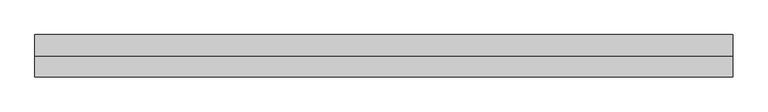
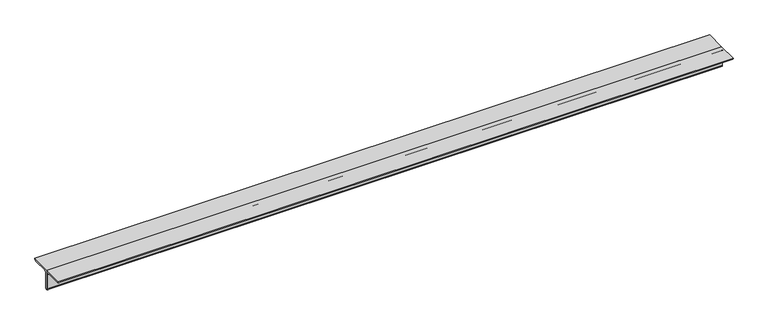
"""IFC4 building model written with IfcOpenShell, lengths in millimetres: member geometry, 0123_Steel Framing_2Ls-KSD3502 : H_SB_AR_S03_2Ls-130x130x12_HBR4."""

import ifcopenshell
import ifcopenshell.guid

model = None  # the IFC model being written
_history = None  # IfcOwnerHistory: only IFC2X3 demands one
_inside = {}  # id of a spatial element -> (the spatial element, [elements in it])
_under = {}  # id of a project, library or spatial element -> (it, [spatial elements below it])
_declared = {}  # id of a project -> (the project, [libraries it declares])
_typed = {}  # id of a type object -> (the type object, [elements of that type])
_made_of = {}  # id of a material, layer set ... -> (it, [elements and type objects made of it])


def new_model(schema):
    """Start an empty IFC model of exactly this schema.

    Asked for "IFC4X3", IfcOpenShell would pick the latest addendum, in which some entities
    have other attributes; the version numbers below select the first issue.
    IFC2X3 requires an IfcOwnerHistory on every rooted entity: one is made here for all.
    """
    global model, _history
    if schema == "IFC4X3":
        model = ifcopenshell.file(schema_version=(4, 3, 0, 0))
    else:
        model = ifcopenshell.file(schema=schema)
    _inside.clear()
    _under.clear()
    _declared.clear()
    _typed.clear()
    _made_of.clear()
    _history = None
    if model.schema == "IFC2X3":
        org = make("IfcOrganization", Name="unknown")
        user = make(
            "IfcPersonAndOrganization",
            ThePerson=make("IfcPerson", FamilyName="unknown"),
            TheOrganization=org,
        )
        app = make(
            "IfcApplication",
            ApplicationDeveloper=org,
            Version="unknown",
            ApplicationFullName="unknown",
            ApplicationIdentifier="unknown",
        )
        _history = make(
            "IfcOwnerHistory",
            OwningUser=user,
            OwningApplication=app,
            ChangeAction="ADDED",
            CreationDate=0,
        )
    return model


def make(cls, **values):
    """One entity of the class cls with the attributes given. An attribute that is None is left unset."""
    return model.create_entity(
        cls, **{name: value for name, value in values.items() if value is not None}
    )


def rooted(cls, **values):
    """An entity with a GlobalId (a new one), such as an element, a storey or a relation."""
    return make(cls, GlobalId=ifcopenshell.guid.new(), OwnerHistory=_history, **values)


def si_unit(unit_type, name, prefix=None):
    """IfcSIUnit, for example si_unit("LENGTHUNIT", "METRE", prefix="MILLI")."""
    return make("IfcSIUnit", UnitType=unit_type, Prefix=prefix, Name=name)


def assignment(units):
    """IfcUnitAssignment: the units of a project."""
    return None if units is None else make("IfcUnitAssignment", Units=units)


def point(xyz):
    """IfcCartesianPoint."""
    return None if xyz is None else make("IfcCartesianPoint", Coordinates=xyz)


def direction(xyz):
    """IfcDirection."""
    return None if xyz is None else make("IfcDirection", DirectionRatios=xyz)


def frame(location, z_axis=None, x_axis=None):
    """IfcAxis2Placement3D, a coordinate frame: its origin and axes. An axis left out is left unset."""
    return make(
        "IfcAxis2Placement3D",
        Location=point(location),
        Axis=direction(z_axis),
        RefDirection=direction(x_axis),
    )


def frame_2d(location, x_axis=None):
    """IfcAxis2Placement2D, a coordinate frame in the plane: its origin and x axis."""
    return make(
        "IfcAxis2Placement2D", Location=point(location), RefDirection=direction(x_axis)
    )


def origin():
    """The frame at (0, 0, 0) with its axes left unset."""
    return frame((0.0, 0.0, 0.0))


def place(relative_to, where):
    """IfcLocalPlacement: puts the frame where relative to a parent placement (None: the world)."""
    return make(
        "IfcLocalPlacement", PlacementRelTo=relative_to, RelativePlacement=where
    )


def context(
    kind, dimensions, precision=None, world=None, true_north=None, identifier=None
):
    """IfcGeometricRepresentationContext, for example the 3D "Model" context."""
    return make(
        "IfcGeometricRepresentationContext",
        ContextIdentifier=identifier,
        ContextType=kind,
        CoordinateSpaceDimension=dimensions,
        Precision=precision,
        WorldCoordinateSystem=world,
        TrueNorth=true_north,
    )


def project(units=None, contexts=None):
    """IfcProject with its units and contexts."""
    return rooted(
        "IfcProject",
        Name="project",
        RepresentationContexts=contexts,
        UnitsInContext=assignment(units),
    )


def spatial(cls, under=None, at=None, **own):
    """A site, building, storey or space (cls), placed at a placement, below another one or the project."""
    s = rooted(cls, ObjectPlacement=at, **own)
    if under is not None:
        _under.setdefault(under.id(), (under, []))[1].append(s)
    return s


def polyline(points):
    """IfcPolyline through the points."""
    return make("IfcPolyline", Points=[point(p) for p in points])


def circle_curve(where, radius):
    """IfcCircle in the frame where."""
    return make("IfcCircle", Position=where, Radius=radius)


def trimmed(basis, trim1, trim2, sense, master):
    """IfcTrimmedCurve: the piece of a basis curve between two trims."""
    return make(
        "IfcTrimmedCurve",
        BasisCurve=basis,
        Trim1=trim1,
        Trim2=trim2,
        SenseAgreement=sense,
        MasterRepresentation=master,
    )


def segment(curve, same_sense, transition):
    """IfcCompositeCurveSegment."""
    return make(
        "IfcCompositeCurveSegment",
        Transition=transition,
        SameSense=same_sense,
        ParentCurve=curve,
    )


def composite_curve(segments, self_intersect=None):
    """IfcCompositeCurve: segments joined end to end."""
    return make("IfcCompositeCurve", Segments=segments, SelfIntersect=self_intersect)


def outline(outer, holes=None, kind="AREA"):
    """IfcArbitraryClosedProfileDef: a profile drawn as a closed curve; with holes, ...WithVoids."""
    if holes is None:
        return make("IfcArbitraryClosedProfileDef", ProfileType=kind, OuterCurve=outer)
    return make(
        "IfcArbitraryProfileDefWithVoids",
        ProfileType=kind,
        OuterCurve=outer,
        InnerCurves=holes,
    )


def extrude(swept, where, along, depth):
    """IfcExtrudedAreaSolid: the profile swept, set in the frame where, extruded along a direction by depth."""
    return make(
        "IfcExtrudedAreaSolid",
        SweptArea=swept,
        Position=where,
        ExtrudedDirection=direction(along),
        Depth=depth,
    )


def shape(context_of_items, identifier, shape_type, items):
    """IfcShapeRepresentation: the items that make up one representation, for example the "Body"."""
    return make(
        "IfcShapeRepresentation",
        ContextOfItems=context_of_items,
        RepresentationIdentifier=identifier,
        RepresentationType=shape_type,
        Items=items,
    )


def source(mapping_origin, context_of_items, identifier, shape_type, items):
    """IfcRepresentationMap: a shape defined once, which mapped items show again and again."""
    return make(
        "IfcRepresentationMap",
        MappingOrigin=mapping_origin,
        MappedRepresentation=shape(context_of_items, identifier, shape_type, items),
    )


def transform(
    local_origin,
    x_axis=None,
    y_axis=None,
    z_axis=None,
    scale=None,
    scale2=None,
    scale3=None,
    uniform=True,
):
    """IfcCartesianTransformationOperator3D, or its non-uniform kind. x_axis, y_axis, z_axis: its Axis1, 2, 3."""
    if uniform:
        return make(
            "IfcCartesianTransformationOperator3D",
            Axis1=direction(x_axis),
            Axis2=direction(y_axis),
            LocalOrigin=point(local_origin),
            Scale=scale,
            Axis3=direction(z_axis),
        )
    return make(
        "IfcCartesianTransformationOperator3DnonUniform",
        Axis1=direction(x_axis),
        Axis2=direction(y_axis),
        LocalOrigin=point(local_origin),
        Scale=scale,
        Axis3=direction(z_axis),
        Scale2=scale2,
        Scale3=scale3,
    )


def mapped(mapping_source, mapping_target):
    """IfcMappedItem: shows the shape of a source again, moved by a transform."""
    return make(
        "IfcMappedItem", MappingSource=mapping_source, MappingTarget=mapping_target
    )


def made_of(thing, what):
    """Note that an element or type object is made of a material, layer set ...; save() writes the relation."""
    if what is not None:
        _made_of.setdefault(what.id(), (what, []))[1].append(thing)
    return thing


def element(
    cls,
    number,
    at=None,
    inside=None,
    cuts=None,
    type_object=None,
    material=None,
    context=None,
    identifier="Body",
    shape_type=None,
    held_by="IfcProductDefinitionShape",
    body=None,
    shapes=None,
    **own,
):
    """One element of the class cls, such as IfcWall. Its Tag is "e" and its number.

    at: its placement. inside: the storey or other place that contains it. cuts: it is an
    opening in that element (IfcRelVoidsElement). A single representation is given by context,
    identifier, shape_type and body (its items); several are given by shapes. held_by: the class
    of the entity that holds the representations. save() writes the other relations.
    """
    e = rooted(cls, Tag="e%d" % number, ObjectPlacement=at, **own)
    if body is not None:
        shapes = [shape(context, identifier, shape_type, body)]
    if shapes is not None:
        e.Representation = make(held_by, Representations=shapes)
    if inside is not None:
        _inside.setdefault(inside.id(), (inside, []))[1].append(e)
    if cuts is not None:
        rooted(
            "IfcRelVoidsElement", RelatingBuildingElement=cuts, RelatedOpeningElement=e
        )
    if type_object is not None:
        _typed.setdefault(type_object.id(), (type_object, []))[1].append(e)
    return made_of(e, material)


def aggregate(whole, parts):
    """IfcRelAggregates: a whole, such as a stair, and the parts it consists of."""
    return rooted("IfcRelAggregates", RelatingObject=whole, RelatedObjects=parts)


def save(model, path):
    """Write the relations noted so far, then the file.

    IfcRelAggregates (storeys below a building ...), IfcRelContainedInSpatialStructure (elements
    in a storey), IfcRelDefinesByType, IfcRelAssociatesMaterial and IfcRelDeclares: one each for
    every whole, place, type object, material and project.
    """
    for whole, parts in _under.values():
        aggregate(whole, parts)
    for where, things in _inside.values():
        rooted(
            "IfcRelContainedInSpatialStructure",
            RelatedElements=things,
            RelatingStructure=where,
        )
    for kind, things in _typed.values():
        rooted("IfcRelDefinesByType", RelatedObjects=things, RelatingType=kind)
    for what, things in _made_of.values():
        rooted("IfcRelAssociatesMaterial", RelatedObjects=things, RelatingMaterial=what)
    for by, libraries in _declared.values():
        rooted("IfcRelDeclares", RelatingContext=by, RelatedDefinitions=libraries)
    model.write(path)


def member_26d310ba(model_context):
    return source(origin(), model_context, "Body", "SweptSolid", [
        extrude(outline(composite_curve([segment(polyline([(0.0, 36.4), (130.0, 36.4)]), True, "CONTINUOUS"), segment(trimmed(circle_curve(frame_2d((118.0, 36.4)), 12.0), [point((130.0, 36.4))], [point((118.0, 24.4))], False, "CARTESIAN"), True, "CONTINUOUS"), segment(polyline([(118.0, 24.4), (24.0, 24.4)]), True, "CONTINUOUS"), segment(trimmed(circle_curve(frame_2d((24.0, 12.4)), 12.0), [point((24.0, 24.4))], [point((12.0, 12.4))], True, "CARTESIAN"), True, "CONTINUOUS"), segment(polyline([(12.0, 12.4), (12.0, -81.6)]), True, "CONTINUOUS"), segment(trimmed(circle_curve(frame_2d((0.0, -81.6)), 12.0), [point((12.0, -81.6))], [point((0.0, -93.6))], False, "CARTESIAN"), True, "CONTINUOUS"), segment(polyline([(0.0, -93.6), (0.0, 36.4)]), True, "CONTINUOUS")], self_intersect=False)), frame((-2215.9, 0.0, 0.0), z_axis=(1.0, 0.0, 0.0), x_axis=(0.0, 1.0, 0.0)), (0.0, 0.0, 1.0), 4294.8666667),
        extrude(outline(composite_curve([segment(polyline([(0.0, 36.4), (0.0, -93.6)]), True, "CONTINUOUS"), segment(trimmed(circle_curve(frame_2d((0.0, -81.6)), 12.0), [point((0.0, -93.6))], [point((-12.0, -81.6))], False, "CARTESIAN"), True, "CONTINUOUS"), segment(polyline([(-12.0, -81.6), (-12.0, 12.4)]), True, "CONTINUOUS"), segment(trimmed(circle_curve(frame_2d((-24.0, 12.4)), 12.0), [point((-12.0, 12.4))], [point((-24.0, 24.4))], True, "CARTESIAN"), True, "CONTINUOUS"), segment(polyline([(-24.0, 24.4), (-118.0, 24.4)]), True, "CONTINUOUS"), segment(trimmed(circle_curve(frame_2d((-118.0, 36.4)), 12.0), [point((-118.0, 24.4))], [point((-130.0, 36.4))], False, "CARTESIAN"), True, "CONTINUOUS"), segment(polyline([(-130.0, 36.4), (0.0, 36.4)]), True, "CONTINUOUS")], self_intersect=False)), frame((-2215.9, 0.0, 0.0), z_axis=(1.0, 0.0, 0.0), x_axis=(0.0, 1.0, 0.0)), (0.0, 0.0, 1.0), 4294.8666667),
    ])


if __name__ == "__main__":
    model = new_model("IFC4")
    model_context = context("Model", 3, world=origin())
    ifc_project = project(units=[si_unit("LENGTHUNIT", "METRE", prefix="MILLI")], contexts=[model_context])
    site = spatial("IfcSite", under=ifc_project)
    building = spatial("IfcBuilding", under=site)
    placement = place(None, origin())
    member_shape = member_26d310ba(model_context)
    element("IfcMember", 1, ObjectType="0123_Steel Framing_2Ls-KSD3502 : H_SB_AR_S03_2Ls-130x130x12_HBR4", at=placement, inside=building, context=model_context, shape_type="MappedRepresentation", body=[
        mapped(member_shape, transform((0.0, 0.0, 0.0), x_axis=(1.0, 0.0, 0.0), y_axis=(0.0, 1.0, 0.0), z_axis=(0.0, 0.0, 1.0))),
    ])
    save(model, "model.ifc")

# Revit data of these elements
# Type "0123_Steel Framing_2Ls-KSD3502 : H_SB_AR_S03_2Ls-130x130x12_HBR4"
#   Type Mark = "HBR4"
#   Assembly Code = "B10"
#   Legs = "SLBB"
#   W = 8.97
#   Perimeter = 1.04 m²/m
#   Nominal Weight = 46.80 kgf/m
#   Length [instance default] = 1000 mm
#   Space = 0 mm
#   b = 130 mm
#   d = 130 mm
#   t = 12 mm
#   y = 36.4 mm
#   A = 0.005952 m²
#   Structural Material [instance default] = Steel ASTM A36
# Element 1 (IfcMember, "0123_Steel Framing_2Ls-KSD3502 : H_SB_AR_S03_2Ls-130x130x12_HBR4")
#   Materials on its faces: "Steel ASTM A36"
# Materials
#   "Steel ASTM A36": class "Metal", colour RGB 199 199 199, transparency 0, Description = "Structural steel, ASTM A36 Grade B, mill finish", Cost = 0
